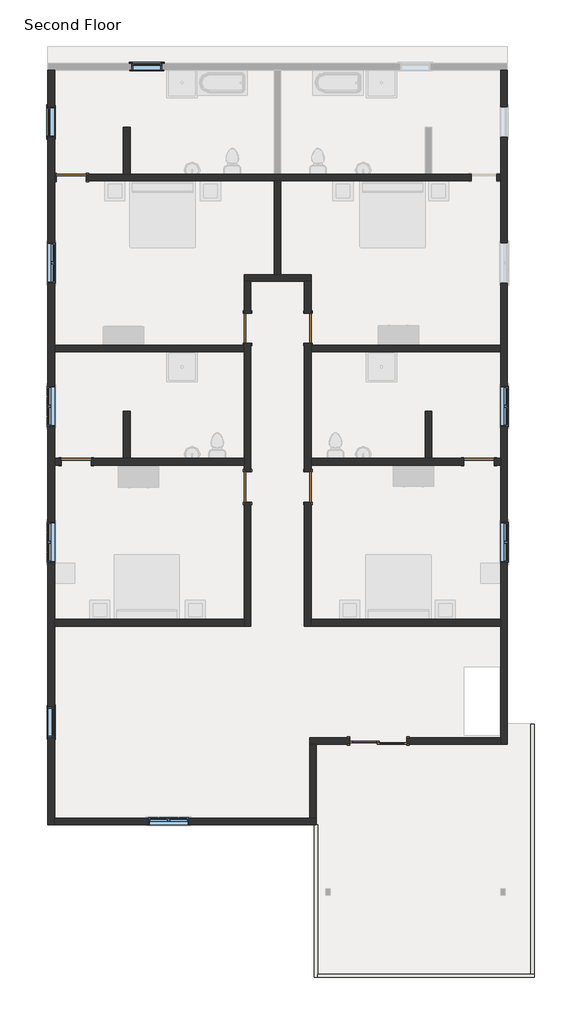
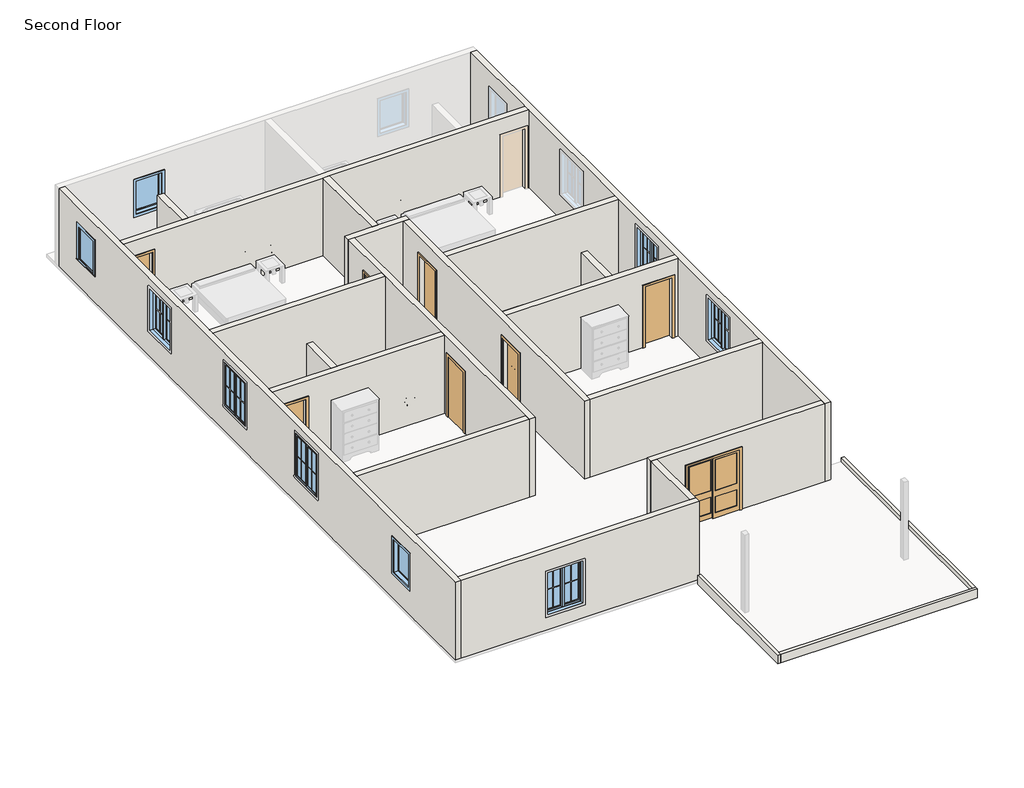
# One storey, part 1 of 2: 22 walls, 9 windows, 8 doors.
"""IFC4 building model written with IfcOpenShell, lengths in millimetres."""

import ifcopenshell
import ifcopenshell.guid

model = None  # the IFC model being written
_history = None  # IfcOwnerHistory: only IFC2X3 demands one
_inside = {}  # id of a spatial element -> (the spatial element, [elements in it])
_under = {}  # id of a project, library or spatial element -> (it, [spatial elements below it])
_declared = {}  # id of a project -> (the project, [libraries it declares])
_typed = {}  # id of a type object -> (the type object, [elements of that type])
_made_of = {}  # id of a material, layer set ... -> (it, [elements and type objects made of it])


def new_model(schema):
    """Start an empty IFC model of exactly this schema.

    Asked for "IFC4X3", IfcOpenShell would pick the latest addendum, in which some entities
    have other attributes; the version numbers below select the first issue.
    IFC2X3 requires an IfcOwnerHistory on every rooted entity: one is made here for all.
    """
    global model, _history
    if schema == "IFC4X3":
        model = ifcopenshell.file(schema_version=(4, 3, 0, 0))
    else:
        model = ifcopenshell.file(schema=schema)
    _inside.clear()
    _under.clear()
    _declared.clear()
    _typed.clear()
    _made_of.clear()
    _history = None
    if model.schema == "IFC2X3":
        org = make("IfcOrganization", Name="unknown")
        user = make(
            "IfcPersonAndOrganization",
            ThePerson=make("IfcPerson", FamilyName="unknown"),
            TheOrganization=org,
        )
        app = make(
            "IfcApplication",
            ApplicationDeveloper=org,
            Version="unknown",
            ApplicationFullName="unknown",
            ApplicationIdentifier="unknown",
        )
        _history = make(
            "IfcOwnerHistory",
            OwningUser=user,
            OwningApplication=app,
            ChangeAction="ADDED",
            CreationDate=0,
        )
    return model


def make(cls, **values):
    """One entity of the class cls with the attributes given. An attribute that is None is left unset."""
    return model.create_entity(
        cls, **{name: value for name, value in values.items() if value is not None}
    )


def rooted(cls, **values):
    """An entity with a GlobalId (a new one), such as an element, a storey or a relation."""
    return make(cls, GlobalId=ifcopenshell.guid.new(), OwnerHistory=_history, **values)


def si_unit(unit_type, name, prefix=None):
    """IfcSIUnit, for example si_unit("LENGTHUNIT", "METRE", prefix="MILLI")."""
    return make("IfcSIUnit", UnitType=unit_type, Prefix=prefix, Name=name)


def assignment(units):
    """IfcUnitAssignment: the units of a project."""
    return None if units is None else make("IfcUnitAssignment", Units=units)


def point(xyz):
    """IfcCartesianPoint."""
    return None if xyz is None else make("IfcCartesianPoint", Coordinates=xyz)


def direction(xyz):
    """IfcDirection."""
    return None if xyz is None else make("IfcDirection", DirectionRatios=xyz)


def frame(location, z_axis=None, x_axis=None):
    """IfcAxis2Placement3D, a coordinate frame: its origin and axes. An axis left out is left unset."""
    return make(
        "IfcAxis2Placement3D",
        Location=point(location),
        Axis=direction(z_axis),
        RefDirection=direction(x_axis),
    )


def origin():
    """The frame at (0, 0, 0) with its axes left unset."""
    return frame((0.0, 0.0, 0.0))


def origin_with_axes():
    """The frame at (0, 0, 0) with the z axis (0, 0, 1) and the x axis (1, 0, 0) written out."""
    return frame((0.0, 0.0, 0.0), z_axis=(0.0, 0.0, 1.0), x_axis=(1.0, 0.0, 0.0))


def place(relative_to, where):
    """IfcLocalPlacement: puts the frame where relative to a parent placement (None: the world)."""
    return make(
        "IfcLocalPlacement", PlacementRelTo=relative_to, RelativePlacement=where
    )


def context(
    kind, dimensions, precision=None, world=None, true_north=None, identifier=None
):
    """IfcGeometricRepresentationContext, for example the 3D "Model" context."""
    return make(
        "IfcGeometricRepresentationContext",
        ContextIdentifier=identifier,
        ContextType=kind,
        CoordinateSpaceDimension=dimensions,
        Precision=precision,
        WorldCoordinateSystem=world,
        TrueNorth=true_north,
    )


def project(units=None, contexts=None):
    """IfcProject with its units and contexts."""
    return rooted(
        "IfcProject",
        Name="project",
        RepresentationContexts=contexts,
        UnitsInContext=assignment(units),
    )


def spatial(cls, under=None, at=None, **own):
    """A site, building, storey or space (cls), placed at a placement, below another one or the project."""
    s = rooted(cls, ObjectPlacement=at, **own)
    if under is not None:
        _under.setdefault(under.id(), (under, []))[1].append(s)
    return s


def polyline(points):
    """IfcPolyline through the points."""
    return make("IfcPolyline", Points=[point(p) for p in points])


def outline(outer, holes=None, kind="AREA"):
    """IfcArbitraryClosedProfileDef: a profile drawn as a closed curve; with holes, ...WithVoids."""
    if holes is None:
        return make("IfcArbitraryClosedProfileDef", ProfileType=kind, OuterCurve=outer)
    return make(
        "IfcArbitraryProfileDefWithVoids",
        ProfileType=kind,
        OuterCurve=outer,
        InnerCurves=holes,
    )


def extrude(swept, where, along, depth):
    """IfcExtrudedAreaSolid: the profile swept, set in the frame where, extruded along a direction by depth."""
    return make(
        "IfcExtrudedAreaSolid",
        SweptArea=swept,
        Position=where,
        ExtrudedDirection=direction(along),
        Depth=depth,
    )


def faces_of(points, faces, orient=None, outer=None):
    """IfcFace entities. A face is a list of loops; a loop is a list of indices into points, from 0.

    orient and outer hold one flag for each loop. By default every Orientation is true, the
    first loop of a face is its IfcFaceOuterBound and the others are IfcFaceBound.
    """
    made = []
    for i, loops in enumerate(faces):
        bounds = []
        for j, loop in enumerate(loops):
            is_outer = j == 0 if outer is None else outer[i][j]
            bounds.append(
                make(
                    "IfcFaceOuterBound" if is_outer else "IfcFaceBound",
                    Bound=make("IfcPolyLoop", Polygon=[points[k] for k in loop]),
                    Orientation=True if orient is None else orient[i][j],
                )
            )
        made.append(make("IfcFace", Bounds=bounds))
    return made


def faceted_brep(points, faces, orient=None, outer=None, voids=None):
    """IfcFacetedBrep: a solid bounded by flat faces; with voids (closed shells), ...WithVoids."""
    shared = [point(p) for p in points]
    hull = make("IfcClosedShell", CfsFaces=faces_of(shared, faces, orient, outer))
    if voids is None:
        return make("IfcFacetedBrep", Outer=hull)
    return make(
        "IfcFacetedBrepWithVoids",
        Outer=hull,
        Voids=[
            make(cls, CfsFaces=faces_of(shared, fs, o, b)) for cls, fs, o, b in voids
        ],
    )


def shape(context_of_items, identifier, shape_type, items):
    """IfcShapeRepresentation: the items that make up one representation, for example the "Body"."""
    return make(
        "IfcShapeRepresentation",
        ContextOfItems=context_of_items,
        RepresentationIdentifier=identifier,
        RepresentationType=shape_type,
        Items=items,
    )


def source(mapping_origin, context_of_items, identifier, shape_type, items):
    """IfcRepresentationMap: a shape defined once, which mapped items show again and again."""
    return make(
        "IfcRepresentationMap",
        MappingOrigin=mapping_origin,
        MappedRepresentation=shape(context_of_items, identifier, shape_type, items),
    )


def transform(
    local_origin,
    x_axis=None,
    y_axis=None,
    z_axis=None,
    scale=None,
    scale2=None,
    scale3=None,
    uniform=True,
):
    """IfcCartesianTransformationOperator3D, or its non-uniform kind. x_axis, y_axis, z_axis: its Axis1, 2, 3."""
    if uniform:
        return make(
            "IfcCartesianTransformationOperator3D",
            Axis1=direction(x_axis),
            Axis2=direction(y_axis),
            LocalOrigin=point(local_origin),
            Scale=scale,
            Axis3=direction(z_axis),
        )
    return make(
        "IfcCartesianTransformationOperator3DnonUniform",
        Axis1=direction(x_axis),
        Axis2=direction(y_axis),
        LocalOrigin=point(local_origin),
        Scale=scale,
        Axis3=direction(z_axis),
        Scale2=scale2,
        Scale3=scale3,
    )


def mapped(mapping_source, mapping_target):
    """IfcMappedItem: shows the shape of a source again, moved by a transform."""
    return make(
        "IfcMappedItem", MappingSource=mapping_source, MappingTarget=mapping_target
    )


def made_of(thing, what):
    """Note that an element or type object is made of a material, layer set ...; save() writes the relation."""
    if what is not None:
        _made_of.setdefault(what.id(), (what, []))[1].append(thing)
    return thing


def element(
    cls,
    number,
    at=None,
    inside=None,
    cuts=None,
    type_object=None,
    material=None,
    context=None,
    identifier="Body",
    shape_type=None,
    held_by="IfcProductDefinitionShape",
    body=None,
    shapes=None,
    **own,
):
    """One element of the class cls, such as IfcWall. Its Tag is "e" and its number.

    at: its placement. inside: the storey or other place that contains it. cuts: it is an
    opening in that element (IfcRelVoidsElement). A single representation is given by context,
    identifier, shape_type and body (its items); several are given by shapes. held_by: the class
    of the entity that holds the representations. save() writes the other relations.
    """
    e = rooted(cls, Tag="e%d" % number, ObjectPlacement=at, **own)
    if body is not None:
        shapes = [shape(context, identifier, shape_type, body)]
    if shapes is not None:
        e.Representation = make(held_by, Representations=shapes)
    if inside is not None:
        _inside.setdefault(inside.id(), (inside, []))[1].append(e)
    if cuts is not None:
        rooted(
            "IfcRelVoidsElement", RelatingBuildingElement=cuts, RelatedOpeningElement=e
        )
    if type_object is not None:
        _typed.setdefault(type_object.id(), (type_object, []))[1].append(e)
    return made_of(e, material)


def aggregate(whole, parts):
    """IfcRelAggregates: a whole, such as a stair, and the parts it consists of."""
    return rooted("IfcRelAggregates", RelatingObject=whole, RelatedObjects=parts)


def save(model, path):
    """Write the relations noted so far, then the file.

    IfcRelAggregates (storeys below a building ...), IfcRelContainedInSpatialStructure (elements
    in a storey), IfcRelDefinesByType, IfcRelAssociatesMaterial and IfcRelDeclares: one each for
    every whole, place, type object, material and project.
    """
    for whole, parts in _under.values():
        aggregate(whole, parts)
    for where, things in _inside.values():
        rooted(
            "IfcRelContainedInSpatialStructure",
            RelatedElements=things,
            RelatingStructure=where,
        )
    for kind, things in _typed.values():
        rooted("IfcRelDefinesByType", RelatedObjects=things, RelatingType=kind)
    for what, things in _made_of.values():
        rooted("IfcRelAssociatesMaterial", RelatedObjects=things, RelatingMaterial=what)
    for by, libraries in _declared.values():
        rooted("IfcRelDeclares", RelatingContext=by, RelatedDefinitions=libraries)
    model.write(path)


def door_54dd4da4(model_context):
    return source(origin(), model_context, "Body", "SweptSolid", [
        extrude(outline(polyline([(2209.8, -533.4), (0.0, -533.4), (0.0, -457.2), (2133.6, -457.2), (2133.6, 457.2), (0.0, 457.2), (0.0, 533.4), (2209.8, 533.4), (2209.8, -533.4)])), frame((0.0, 101.6, 0.0), z_axis=(0.0, 1.0, 0.0), x_axis=(0.0, 0.0, 1.0)), (0.0, 0.0, 1.0), 25.4),
        extrude(outline(polyline([(2209.8, 533.4), (2209.8, -533.4), (0.0, -533.4), (0.0, -457.2), (2133.6, -457.2), (2133.6, 457.2), (0.0, 457.2), (0.0, 533.4), (2209.8, 533.4)])), frame((0.0, -127.0, 0.0), z_axis=(0.0, 1.0, 0.0), x_axis=(0.0, 0.0, 1.0)), (0.0, 0.0, 1.0), 25.4),
        extrude(outline(polyline([(457.2, 50.8), (-457.2, 50.8), (-457.2, 101.6), (457.2, 101.6), (457.2, 50.8)])), origin_with_axes(), (0.0, 0.0, 1.0), 2133.6),
    ])


def door_719f80de(model_context):
    return source(origin(), model_context, "Body", "SweptSolid", [
        extrude(outline(polyline([(2209.8, -533.4), (0.0, -533.4), (0.0, -457.2), (2133.6, -457.2), (2133.6, 457.2), (0.0, 457.2), (0.0, 533.4), (2209.8, 533.4), (2209.8, -533.4)])), frame((0.0, -127.0, 0.0), z_axis=(0.0, 1.0, 0.0), x_axis=(0.0, 0.0, 1.0)), (0.0, 0.0, 1.0), 25.4),
        extrude(outline(polyline([(2209.8, 533.4), (2209.8, -533.4), (0.0, -533.4), (0.0, -457.2), (2133.6, -457.2), (2133.6, 457.2), (0.0, 457.2), (0.0, 533.4), (2209.8, 533.4)])), frame((0.0, 101.6, 0.0), z_axis=(0.0, 1.0, 0.0), x_axis=(0.0, 0.0, 1.0)), (0.0, 0.0, 1.0), 25.4),
        extrude(outline(polyline([(457.2, -50.8), (457.2, -101.6), (-457.2, -101.6), (-457.2, -50.8), (457.2, -50.8)])), origin_with_axes(), (0.0, 0.0, 1.0), 2133.6),
    ])


def door_2f313a91(model_context):
    return source(origin(), model_context, "Body", "SweptSolid", [
        extrude(outline(polyline([(-63.5, 190.5), (-774.7, 190.5), (-774.7, 215.9), (-63.5, 215.9), (-63.5, 190.5)])), frame((0.0, 0.0, 965.2), z_axis=(0.0, 0.0, 1.0), x_axis=(1.0, 0.0, 0.0)), (0.0, 0.0, 1.0), 1079.5),
        extrude(outline(polyline([(-63.5, 190.5), (-774.7, 190.5), (-774.7, 215.9), (-63.5, 215.9), (-63.5, 190.5)])), frame((0.0, 0.0, 184.15), z_axis=(0.0, 0.0, 1.0), x_axis=(1.0, 0.0, 0.0)), (0.0, 0.0, 1.0), 565.15),
        extrude(outline(polyline([(63.5, 165.1), (774.7, 165.1), (774.7, 139.7), (63.5, 139.7), (63.5, 165.1)])), frame((0.0, 0.0, 965.2), z_axis=(0.0, 0.0, 1.0), x_axis=(1.0, 0.0, 0.0)), (0.0, 0.0, 1.0), 1079.5),
        extrude(outline(polyline([(63.5, 165.1), (774.7, 165.1), (774.7, 139.7), (63.5, 139.7), (63.5, 165.1)])), frame((0.0, 0.0, 184.15), z_axis=(0.0, 0.0, 1.0), x_axis=(1.0, 0.0, 0.0)), (0.0, 0.0, 1.0), 565.15),
        extrude(outline(polyline([(2133.6, 25.4), (2133.6, -863.6), (0.0, -863.6), (0.0, 25.4), (2133.6, 25.4)]), holes=[polyline([(184.15, -774.7), (749.3, -774.7), (749.3, -63.5), (184.15, -63.5), (184.15, -774.7)]), polyline([(965.2, -774.7), (2044.7, -774.7), (2044.7, -63.5), (965.2, -63.5), (965.2, -774.7)])]), frame((0.0, 177.8, 0.0), z_axis=(0.0, 1.0, 0.0), x_axis=(0.0, 0.0, 1.0)), (0.0, 0.0, 1.0), 50.8),
        extrude(outline(polyline([(0.0, -939.8), (0.0, -863.6), (2133.6, -863.6), (2133.6, 863.6), (0.0, 863.6), (0.0, 939.8), (2209.8, 939.8), (2209.8, -939.8), (0.0, -939.8)])), frame((0.0, 0.0, 0.0), z_axis=(0.0, 1.0, 0.0), x_axis=(0.0, 0.0, 1.0)), (0.0, 0.0, 1.0), 25.4),
        extrude(outline(polyline([(0.0, 939.8), (2209.8, 939.8), (2209.8, -939.8), (0.0, -939.8), (0.0, -863.6), (2133.6, -863.6), (2133.6, 863.6), (0.0, 863.6), (0.0, 939.8)])), frame((0.0, 228.6, 0.0), z_axis=(0.0, 1.0, 0.0), x_axis=(0.0, 0.0, 1.0)), (0.0, 0.0, 1.0), 25.4),
        extrude(outline(polyline([(2133.6, -25.4), (0.0, -25.4), (0.0, 863.6), (2133.6, 863.6), (2133.6, -25.4)]), holes=[polyline([(965.2, 774.7), (965.2, 63.5), (2044.7, 63.5), (2044.7, 774.7), (965.2, 774.7)]), polyline([(184.15, 774.7), (184.15, 63.5), (749.3, 63.5), (749.3, 774.7), (184.15, 774.7)])]), frame((0.0, 127.0, 0.0), z_axis=(0.0, 1.0, 0.0), x_axis=(0.0, 0.0, 1.0)), (0.0, 0.0, 1.0), 50.8),
    ])


def window_bec2521a(model_context):
    return source(origin(), model_context, "Body", "SweptSolid", [
        extrude(outline(polyline([(-565.15, 127.0), (488.95, 127.0), (488.95, 101.6), (-565.15, 101.6), (-565.15, 127.0)])), frame((0.0, 0.0, 914.4), z_axis=(0.0, 0.0, 1.0), x_axis=(1.0, 0.0, 0.0)), (0.0, 0.0, 1.0), 19.05),
        extrude(outline(polyline([(2114.55, -476.25), (2114.55, 400.05), (933.45, 400.05), (933.45, 488.95), (2203.45, 488.95), (2203.45, -565.15), (933.45, -565.15), (933.45, -476.25), (2114.55, -476.25)])), frame((0.0, 101.6, 0.0), z_axis=(0.0, 1.0, 0.0), x_axis=(0.0, 0.0, 1.0)), (0.0, 0.0, 1.0), 12.7),
        extrude(outline(polyline([(2190.75, 476.25), (2190.75, -552.45), (857.25, -552.45), (857.25, 476.25), (2190.75, 476.25)]), holes=[polyline([(2101.85, 387.35), (946.15, 387.35), (946.15, -463.55), (2101.85, -463.55), (2101.85, 387.35)])]), frame((0.0, -120.65, 0.0), z_axis=(0.0, 1.0, 0.0), x_axis=(0.0, 0.0, 1.0)), (0.0, 0.0, 1.0), 19.05),
        extrude(outline(polyline([(355.6, 53.975), (-431.8, 53.975), (-431.8, 66.675), (355.6, 66.675), (355.6, 53.975)])), frame((0.0, 0.0, 977.9), z_axis=(0.0, 0.0, 1.0), x_axis=(1.0, 0.0, 0.0)), (0.0, 0.0, 1.0), 1092.2),
        extrude(outline(polyline([(2114.55, -476.25), (933.45, -476.25), (933.45, 400.05), (2114.55, 400.05), (2114.55, -476.25)]), holes=[polyline([(2070.1, -431.8), (2070.1, 355.6), (977.9, 355.6), (977.9, -431.8), (2070.1, -431.8)])]), frame((0.0, 38.1, 0.0), z_axis=(0.0, 1.0, 0.0), x_axis=(0.0, 0.0, 1.0)), (0.0, 0.0, 1.0), 44.45),
        extrude(outline(polyline([(2133.6, -495.3), (914.4, -495.3), (914.4, 419.1), (2133.6, 419.1), (2133.6, -495.3)]), holes=[polyline([(2101.85, -463.55), (2101.85, 387.35), (946.15, 387.35), (946.15, -463.55), (2101.85, -463.55)])]), frame((0.0, -101.6, 0.0), z_axis=(0.0, 1.0, 0.0), x_axis=(0.0, 0.0, 1.0)), (0.0, 0.0, 1.0), 139.7),
        extrude(outline(polyline([(2133.6, 419.1), (2133.6, -495.3), (914.4, -495.3), (914.4, 419.1), (2133.6, 419.1)]), holes=[polyline([(2114.55, 400.05), (933.45, 400.05), (933.45, -476.25), (2114.55, -476.25), (2114.55, 400.05)])]), frame((0.0, 38.1, 0.0), z_axis=(0.0, 1.0, 0.0), x_axis=(0.0, 0.0, 1.0)), (0.0, 0.0, 1.0), 63.5),
    ])


def window_78633f8a(model_context):
    return source(origin(), model_context, "Body", "SolidModel", [
        faceted_brep([(9.525, 120.65, 2425.7), (-9.525, 120.65, 2425.7), (-9.525, 69.85, 2425.7), (9.525, 69.85, 2425.7), (9.525, 120.65, 927.1), (9.525, 69.85, 927.1), (-9.525, 69.85, 927.1), (-9.525, 120.65, 927.1), (-9.525, 69.85, 946.15), (-9.525, 69.85, 2406.65), (-30.1625, 69.85, 946.15), (-30.1625, 69.85, 2406.65), (-30.1625, 6.35, 946.15), (-30.1625, 6.35, 2406.65), (30.1625, 6.35, 946.15), (30.1625, 6.35, 2406.65), (30.1625, 69.85, 946.15), (30.1625, 69.85, 2406.65), (9.525, 69.85, 946.15), (9.525, 69.85, 2406.65)], [[[0, 1, 2, 3]], [[4, 5, 6, 7]], [[1, 0, 4, 7]], [[2, 1, 7, 6, 8, 9]], [[9, 8, 10, 11]], [[11, 10, 12, 13]], [[13, 12, 14, 15]], [[15, 14, 16, 17]], [[17, 16, 18, 19]], [[0, 3, 19, 18, 5, 4]], [[18, 8, 6, 5]], [[9, 19, 3, 2]], [[8, 18, 16, 14, 12, 10]], [[19, 9, 11, 13, 15, 17]]]),
        extrude(outline(polyline([(-66.675, 101.6), (-66.675, 95.25), (-539.75, 95.25), (-539.75, 101.6), (-66.675, 101.6)])), frame((0.0, 0.0, 984.25), z_axis=(0.0, 0.0, 1.0), x_axis=(1.0, 0.0, 0.0)), (0.0, 0.0, 1.0), 1384.3),
        extrude(outline(polyline([(-539.75, 82.55), (-539.75, 88.9), (-66.675, 88.9), (-66.675, 82.55), (-539.75, 82.55)])), frame((0.0, 0.0, 984.25), z_axis=(0.0, 0.0, 1.0), x_axis=(1.0, 0.0, 0.0)), (0.0, 0.0, 1.0), 1384.3),
        extrude(outline(polyline([(539.75, 101.6), (539.75, 95.25), (66.675, 95.25), (66.675, 101.6), (539.75, 101.6)])), frame((0.0, 0.0, 984.25), z_axis=(0.0, 0.0, 1.0), x_axis=(1.0, 0.0, 0.0)), (0.0, 0.0, 1.0), 1384.3),
        extrude(outline(polyline([(66.675, 82.55), (66.675, 88.9), (539.75, 88.9), (539.75, 82.55), (66.675, 82.55)])), frame((0.0, 0.0, 984.25), z_axis=(0.0, 0.0, 1.0), x_axis=(1.0, 0.0, 0.0)), (0.0, 0.0, 1.0), 1384.3),
        extrude(outline(polyline([(2425.7, -596.9), (927.1, -596.9), (927.1, -9.525), (2425.7, -9.525), (2425.7, -596.9)]), holes=[polyline([(2368.55, -66.675), (984.25, -66.675), (984.25, -539.75), (2368.55, -539.75), (2368.55, -66.675)])]), frame((0.0, 69.85, 0.0), z_axis=(0.0, 1.0, 0.0), x_axis=(0.0, 0.0, 1.0)), (0.0, 0.0, 1.0), 44.45),
        extrude(outline(polyline([(927.1, 596.9), (2425.7, 596.9), (2425.7, 9.525), (927.1, 9.525), (927.1, 596.9)]), holes=[polyline([(984.25, 66.675), (2368.55, 66.675), (2368.55, 539.75), (984.25, 539.75), (984.25, 66.675)])]), frame((0.0, 69.85, 0.0), z_axis=(0.0, 1.0, 0.0), x_axis=(0.0, 0.0, 1.0)), (0.0, 0.0, 1.0), 44.45),
        extrude(outline(polyline([(2438.4, -609.6), (914.4, -609.6), (914.4, 609.6), (2438.4, 609.6), (2438.4, -609.6)]), holes=[polyline([(2419.35, 590.55), (933.45, 590.55), (933.45, -590.55), (2419.35, -590.55), (2419.35, 590.55)])]), frame((0.0, -101.6, 0.0), z_axis=(0.0, 1.0, 0.0), x_axis=(0.0, 0.0, 1.0)), (0.0, 0.0, 1.0), 107.95),
        faceted_brep([(577.85, 69.85, 2406.65), (577.85, 6.35, 2406.65), (-577.85, 6.35, 2406.65), (-577.85, 69.85, 2406.65), (596.9, 120.65, 2425.7), (596.9, 69.85, 2425.7), (-596.9, 69.85, 2425.7), (-596.9, 120.65, 2425.7), (609.6, 6.35, 2438.4), (609.6, 120.65, 2438.4), (-609.6, 120.65, 2438.4), (-609.6, 6.35, 2438.4), (-577.85, 6.35, 946.15), (-577.85, 69.85, 946.15), (-596.9, 69.85, 927.1), (-596.9, 120.65, 927.1), (-609.6, 120.65, 914.4), (-609.6, 6.35, 914.4), (577.85, 6.35, 946.15), (577.85, 69.85, 946.15), (596.9, 69.85, 927.1), (596.9, 120.65, 927.1), (609.6, 120.65, 914.4), (609.6, 6.35, 914.4)], [[[0, 1, 2, 3]], [[4, 5, 6, 7]], [[8, 9, 10, 11]], [[3, 2, 12, 13]], [[7, 6, 14, 15]], [[11, 10, 16, 17]], [[13, 12, 18, 19]], [[15, 14, 20, 21]], [[17, 16, 22, 23]], [[11, 17, 23, 8], [1, 18, 12, 2]], [[19, 18, 1, 0]], [[5, 20, 14, 6], [3, 13, 19, 0]], [[21, 20, 5, 4]], [[23, 22, 9, 8]], [[9, 22, 16, 10], [7, 15, 21, 4]]]),
    ])


model = new_model("IFC4")

# Units and contexts
model_context = context("Model", 3, world=origin())
ifc_project = project(units=[si_unit("LENGTHUNIT", "METRE", prefix="MILLI")], contexts=[model_context])

# Site, building, storey
site = spatial("IfcSite", under=ifc_project)
building = spatial("IfcBuilding", under=site)
storey = spatial("IfcBuildingStorey", under=building, Name="Second Floor", Elevation=2743.2)

# Doors
placement = place(None, origin())
door_shape = door_54dd4da4(model_context)
element("IfcDoor", 1, ObjectType="Single-Flush : 36\" x 84\"", at=placement, inside=storey, context=model_context, shape_type="MappedRepresentation", body=[
    mapped(door_shape, transform((-5575.1210655, 3585.6263295, 2743.2), x_axis=(1.0, 0.0, 0.0), y_axis=(0.0, 1.0, 0.0), z_axis=(0.0, 0.0, 1.0))),
])
element("IfcDoor", 2, ObjectType="Single-Flush : 36\" x 84\"", at=placement, inside=storey, context=model_context, shape_type="MappedRepresentation", body=[
    mapped(door_shape, transform((1587.6789345, -986.3736705, 2743.2), x_axis=(0.0, -1.0, 0.0), y_axis=(1.0, 0.0, 0.0), z_axis=(0.0, 0.0, 1.0))),
])
element("IfcDoor", 3, ObjectType="Single-Flush : 36\" x 84\"", at=placement, inside=storey, context=model_context, shape_type="MappedRepresentation", body=[
    mapped(door_shape, transform((-5422.7210655, -5024.9736705, 2743.2), x_axis=(1.0, 0.0, 0.0), y_axis=(0.0, 1.0, 0.0), z_axis=(0.0, 0.0, 1.0))),
])
element("IfcDoor", 4, ObjectType="Single-Flush : 36\" x 84\"", at=placement, inside=storey, context=model_context, shape_type="MappedRepresentation", body=[
    mapped(door_shape, transform((-241.1210655, -5786.9736705, 2743.2), x_axis=(0.0, 1.0, 0.0), y_axis=(-1.0, 0.0, 0.0), z_axis=(0.0, 0.0, 1.0))),
])
door_2_shape = door_719f80de(model_context)
element("IfcDoor", 5, ObjectType="Single-Flush : 36\" x 84\"", at=placement, inside=storey, context=model_context, shape_type="MappedRepresentation", body=[
    mapped(door_2_shape, transform((6769.2789345, -5024.9736705, 2743.2), x_axis=(-1.0, 0.0, 0.0), y_axis=(0.0, -1.0, 0.0), z_axis=(0.0, 0.0, 1.0))),
])
element("IfcDoor", 6, ObjectType="Single-Flush : 36\" x 84\"", at=placement, inside=storey, context=model_context, shape_type="MappedRepresentation", body=[
    mapped(door_2_shape, transform((-241.1210655, -986.3736705, 2743.2), x_axis=(0.0, -1.0, 0.0), y_axis=(1.0, 0.0, 0.0), z_axis=(0.0, 0.0, 1.0))),
])
element("IfcDoor", 7, ObjectType="Single-Flush : 36\" x 84\"", at=placement, inside=storey, context=model_context, shape_type="MappedRepresentation", body=[
    mapped(door_2_shape, transform((1587.6789345, -5786.9736705, 2743.2), x_axis=(0.0, 1.0, 0.0), y_axis=(-1.0, 0.0, 0.0), z_axis=(0.0, 0.0, 1.0))),
])
door_3_shape = door_2f313a91(model_context)
element("IfcDoor", 8, ObjectType="Sliding-Closet : 68\" x 84\"", at=placement, inside=storey, context=model_context, shape_type="MappedRepresentation", body=[
    mapped(door_3_shape, transform((3721.2789345, -13356.1736705, 2743.2), x_axis=(-1.0, 0.0, 0.0), y_axis=(0.0, -1.0, 0.0), z_axis=(0.0, 0.0, 1.0))),
])

# Walls
element("IfcWall", 9, ObjectType="Generic - 4\"", at=placement, inside=storey, context=model_context, shape_type="Brep", body=[
    faceted_brep([(1786.1164345, -16023.1736705, 2590.8), (1786.1164345, -20641.2111705, 2590.8), (1786.1164345, -20641.2111705, 2895.6), (1786.1164345, -16023.1736705, 2895.6), (1887.7164345, -16023.1736705, 2590.8), (1887.7164345, -16023.1736705, 2895.6), (1887.7164345, -20539.6111705, 2895.6), (1887.7164345, -20641.2111705, 2895.6), (1887.7164345, -20641.2111705, 2590.8), (1887.7164345, -20539.6111705, 2590.8)], [[[0, 1, 2, 3]], [[4, 5, 6, 7, 8, 9]], [[1, 0, 4, 9, 8]], [[3, 2, 7, 6, 5]], [[0, 3, 5, 4]], [[2, 1, 8, 7]]]),
])
element("IfcWall", 10, ObjectType="Generic - 4\"", at=placement, inside=storey, context=model_context, shape_type="Brep", body=[
    faceted_brep([(1887.7164345, -20641.2111705, 2590.8), (8440.9164345, -20641.2111705, 2590.8), (8440.9164345, -20641.2111705, 2895.6), (1887.7164345, -20641.2111705, 2895.6), (1887.7164345, -20539.6111705, 2590.8), (1887.7164345, -20539.6111705, 2895.6), (8339.3164345, -20539.6111705, 2895.6), (8440.9164345, -20539.6111705, 2895.6), (8440.9164345, -20539.6111705, 2590.8), (8339.3164345, -20539.6111705, 2590.8)], [[[0, 1, 2, 3]], [[4, 5, 6, 7, 8, 9]], [[1, 0, 4, 9, 8]], [[3, 2, 7, 6, 5]], [[0, 3, 5, 4]], [[2, 1, 8, 7]]]),
])
element("IfcWall", 11, ObjectType="Generic - 4\"", at=placement, inside=storey, context=model_context, shape_type="SweptSolid", body=[
    extrude(outline(polyline([(8440.9164345, -12970.4111705), (8440.9164345, -20539.6111705), (8339.3164345, -20539.6111705), (8339.3164345, -12970.4111705), (8440.9164345, -12970.4111705)])), frame((0.0, 0.0, 2590.8), z_axis=(0.0, 0.0, 1.0), x_axis=(1.0, 0.0, 0.0)), (0.0, 0.0, 1.0), 304.8),
])
element("IfcWall", 12, ObjectType="Generic - 8\" - Filled", at=placement, inside=storey, context=model_context, shape_type="Brep", body=[
    faceted_brep([(7429.6789345, 6836.8263295, 2743.2), (7429.6789345, 3687.2263295, 2743.2), (7429.6789345, 3484.0263295, 2743.2), (7429.6789345, -1494.3736705, 2743.2), (7429.6789345, -1697.5736705, 2743.2), (7429.6789345, -4923.3736705, 2743.2), (7429.6789345, -5126.5736705, 2743.2), (7429.6789345, -9800.1736705, 2743.2), (7429.6789345, -10003.3736705, 2743.2), (7429.6789345, -13381.5736705, 2743.2), (7429.6789345, -13584.7736705, 2743.2), (7429.6789345, -13584.7736705, 5486.4), (7429.6789345, -13381.5736705, 5486.4), (7429.6789345, -10003.3736705, 5486.4), (7429.6789345, -9800.1736705, 5486.4), (7429.6789345, -5126.5736705, 5486.4), (7429.6789345, -4923.3736705, 5486.4), (7429.6789345, -1697.5736705, 5486.4), (7429.6789345, -1494.3736705, 5486.4), (7429.6789345, 3484.0263295, 5486.4), (7429.6789345, 3687.2263295, 5486.4), (7429.6789345, 6836.8263295, 5486.4), (7429.6789345, 4804.8263295, 4876.8), (7429.6789345, 4804.8263295, 3657.6), (7429.6789345, 5719.2263295, 3657.6), (7429.6789345, 5719.2263295, 4876.8), (7429.6789345, -3958.1736705, 5181.6), (7429.6789345, -3958.1736705, 3657.6), (7429.6789345, -2738.9736705, 3657.6), (7429.6789345, -2738.9736705, 5181.6), (7429.6789345, -8072.9736705, 5181.6), (7429.6789345, -8072.9736705, 3657.6), (7429.6789345, -6853.7736705, 3657.6), (7429.6789345, -6853.7736705, 5181.6), (7429.6789345, 385.2263295, 5181.6), (7429.6789345, 385.2263295, 3657.6), (7429.6789345, 1604.4263295, 3657.6), (7429.6789345, 1604.4263295, 5181.6), (7632.8789345, 6836.8263295, 2743.2), (7632.8789345, 6836.8263295, 5486.4), (7632.8789345, -13584.7736705, 5486.4), (7632.8789345, -13584.7736705, 2743.2), (7632.8789345, 4804.8263295, 4876.8), (7632.8789345, 5719.2263295, 4876.8), (7632.8789345, 5719.2263295, 3657.6), (7632.8789345, 4804.8263295, 3657.6), (7632.8789345, -3958.1736705, 5181.6), (7632.8789345, -2738.9736705, 5181.6), (7632.8789345, -2738.9736705, 3657.6), (7632.8789345, -3958.1736705, 3657.6), (7632.8789345, -8072.9736705, 5181.6), (7632.8789345, -6853.7736705, 5181.6), (7632.8789345, -6853.7736705, 3657.6), (7632.8789345, -8072.9736705, 3657.6), (7632.8789345, 385.2263295, 5181.6), (7632.8789345, 1604.4263295, 5181.6), (7632.8789345, 1604.4263295, 3657.6), (7632.8789345, 385.2263295, 3657.6)], [[[0, 1, 2, 3, 4, 5, 6, 7, 8, 9, 10, 11, 12, 13, 14, 15, 16, 17, 18, 19, 20, 21], [22, 23, 24, 25], [26, 27, 28, 29], [30, 31, 32, 33], [34, 35, 36, 37]], [[38, 39, 40, 41], [42, 43, 44, 45], [46, 47, 48, 49], [50, 51, 52, 53], [54, 55, 56, 57]], [[10, 9, 8, 7, 6, 5, 4, 3, 2, 1, 0, 38, 41]], [[21, 20, 19, 18, 17, 16, 15, 14, 13, 12, 11, 40, 39]], [[0, 21, 39, 38]], [[23, 22, 42, 45]], [[24, 23, 45, 44]], [[25, 24, 44, 43]], [[22, 25, 43, 42]], [[27, 26, 46, 49]], [[28, 27, 49, 48]], [[29, 28, 48, 47]], [[26, 29, 47, 46]], [[11, 10, 41, 40]], [[31, 30, 50, 53]], [[32, 31, 53, 52]], [[33, 32, 52, 51]], [[30, 33, 51, 50]], [[35, 34, 54, 57]], [[36, 35, 57, 56]], [[37, 36, 56, 55]], [[34, 37, 55, 54]]]),
])
element("IfcWall", 13, ObjectType="Generic - 8\" - Filled", at=placement, inside=storey, context=model_context, shape_type="Brep", body=[
    faceted_brep([(-6083.1210655, -16023.1736705, 2743.2), (-6083.1210655, -15819.9736705, 2743.2), (-6083.1210655, -10003.3736705, 2743.2), (-6083.1210655, -9800.1736705, 2743.2), (-6083.1210655, -5126.5736705, 2743.2), (-6083.1210655, -4923.3736705, 2743.2), (-6083.1210655, -1697.5736705, 2743.2), (-6083.1210655, -1494.3736705, 2743.2), (-6083.1210655, 3484.0263295, 2743.2), (-6083.1210655, 3687.2263295, 2743.2), (-6083.1210655, 6836.8263295, 2743.2), (-6083.1210655, 6836.8263295, 5486.4), (-6083.1210655, 3687.2263295, 5486.4), (-6083.1210655, 3484.0263295, 5486.4), (-6083.1210655, -1494.3736705, 5486.4), (-6083.1210655, -1697.5736705, 5486.4), (-6083.1210655, -4923.3736705, 5486.4), (-6083.1210655, -5126.5736705, 5486.4), (-6083.1210655, -9800.1736705, 5486.4), (-6083.1210655, -10003.3736705, 5486.4), (-6083.1210655, -15819.9736705, 5486.4), (-6083.1210655, -16023.1736705, 5486.4), (-6083.1210655, 5719.2263295, 4876.8), (-6083.1210655, 5719.2263295, 3657.6), (-6083.1210655, 4804.8263295, 3657.6), (-6083.1210655, 4804.8263295, 4876.8), (-6083.1210655, -2738.9736705, 5181.6), (-6083.1210655, -2738.9736705, 3657.6), (-6083.1210655, -3958.1736705, 3657.6), (-6083.1210655, -3958.1736705, 5181.6), (-6083.1210655, -6853.7736705, 5181.6), (-6083.1210655, -6853.7736705, 3657.6), (-6083.1210655, -8072.9736705, 3657.6), (-6083.1210655, -8072.9736705, 5181.6), (-6083.1210655, -13368.8736705, 4876.8), (-6083.1210655, -12454.4736705, 4876.8), (-6083.1210655, -12454.4736705, 3657.6), (-6083.1210655, -13368.8736705, 3657.6), (-6083.1210655, 385.2263295, 5181.6), (-6083.1210655, 1604.4263295, 5181.6), (-6083.1210655, 1604.4263295, 3657.6), (-6083.1210655, 385.2263295, 3657.6), (-6286.3210655, -16023.1736705, 2743.2), (-6286.3210655, -16023.1736705, 5486.4), (-6286.3210655, 6836.8263295, 5486.4), (-6286.3210655, 6836.8263295, 2743.2), (-6286.3210655, 5719.2263295, 4876.8), (-6286.3210655, 4804.8263295, 4876.8), (-6286.3210655, 4804.8263295, 3657.6), (-6286.3210655, 5719.2263295, 3657.6), (-6286.3210655, -2738.9736705, 5181.6), (-6286.3210655, -3958.1736705, 5181.6), (-6286.3210655, -3958.1736705, 3657.6), (-6286.3210655, -2738.9736705, 3657.6), (-6286.3210655, -6853.7736705, 5181.6), (-6286.3210655, -8072.9736705, 5181.6), (-6286.3210655, -8072.9736705, 3657.6), (-6286.3210655, -6853.7736705, 3657.6), (-6286.3210655, -13368.8736705, 4876.8), (-6286.3210655, -13368.8736705, 3657.6), (-6286.3210655, -12454.4736705, 3657.6), (-6286.3210655, -12454.4736705, 4876.8), (-6286.3210655, 385.2263295, 5181.6), (-6286.3210655, 385.2263295, 3657.6), (-6286.3210655, 1604.4263295, 3657.6), (-6286.3210655, 1604.4263295, 5181.6)], [[[0, 1, 2, 3, 4, 5, 6, 7, 8, 9, 10, 11, 12, 13, 14, 15, 16, 17, 18, 19, 20, 21], [22, 23, 24, 25], [26, 27, 28, 29], [30, 31, 32, 33], [34, 35, 36, 37], [38, 39, 40, 41]], [[42, 43, 44, 45], [46, 47, 48, 49], [50, 51, 52, 53], [54, 55, 56, 57], [58, 59, 60, 61], [62, 63, 64, 65]], [[10, 9, 8, 7, 6, 5, 4, 3, 2, 1, 0, 42, 45]], [[21, 20, 19, 18, 17, 16, 15, 14, 13, 12, 11, 44, 43]], [[11, 10, 45, 44]], [[23, 22, 46, 49]], [[24, 23, 49, 48]], [[25, 24, 48, 47]], [[22, 25, 47, 46]], [[0, 21, 43, 42]], [[27, 26, 50, 53]], [[28, 27, 53, 52]], [[29, 28, 52, 51]], [[26, 29, 51, 50]], [[31, 30, 54, 57]], [[32, 31, 57, 56]], [[33, 32, 56, 55]], [[30, 33, 55, 54]], [[59, 58, 34, 37]], [[60, 59, 37, 36]], [[61, 60, 36, 35]], [[58, 61, 35, 34]], [[63, 62, 38, 41]], [[64, 63, 41, 40]], [[65, 64, 40, 39]], [[62, 65, 39, 38]]]),
])
element("IfcWall", 14, ObjectType="Generic - 8\" - Filled", at=placement, inside=storey, context=model_context, shape_type="Brep", body=[
    faceted_brep([(-5117.9210655, 3484.0263295, 2743.2), (571.6789345, 3484.0263295, 2743.2), (774.8789345, 3484.0263295, 2743.2), (6540.6789345, 3484.0263295, 2743.2), (6540.6789345, 3484.0263295, 4876.8), (7302.6789345, 3484.0263295, 4876.8), (7302.6789345, 3484.0263295, 2743.2), (7429.6789345, 3484.0263295, 2743.2), (7429.6789345, 3484.0263295, 5486.4), (774.8789345, 3484.0263295, 5486.4), (571.6789345, 3484.0263295, 5486.4), (-6083.1210655, 3484.0263295, 5486.4), (-6083.1210655, 3484.0263295, 2743.2), (-6032.3210655, 3484.0263295, 2743.2), (-6032.3210655, 3484.0263295, 4876.8), (-5117.9210655, 3484.0263295, 4876.8), (6540.6789345, 3687.2263295, 4876.8), (6540.6789345, 3687.2263295, 2743.2), (5346.8789345, 3687.2263295, 2743.2), (5143.6789345, 3687.2263295, 2743.2), (774.8789345, 3687.2263295, 2743.2), (571.6789345, 3687.2263295, 2743.2), (-3797.1210655, 3687.2263295, 2743.2), (-4000.3210655, 3687.2263295, 2743.2), (-5117.9210655, 3687.2263295, 2743.2), (-5117.9210655, 3687.2263295, 4876.8), (-6032.3210655, 3687.2263295, 4876.8), (-6032.3210655, 3687.2263295, 2743.2), (-6083.1210655, 3687.2263295, 2743.2), (-6083.1210655, 3687.2263295, 5486.4), (-4000.3210655, 3687.2263295, 5486.4), (-3797.1210655, 3687.2263295, 5486.4), (571.6789345, 3687.2263295, 5486.4), (774.8789345, 3687.2263295, 5486.4), (5143.6789345, 3687.2263295, 5486.4), (5346.8789345, 3687.2263295, 5486.4), (7429.6789345, 3687.2263295, 5486.4), (7429.6789345, 3687.2263295, 2743.2), (7302.6789345, 3687.2263295, 2743.2), (7302.6789345, 3687.2263295, 4876.8)], [[[0, 1, 2, 3, 4, 5, 6, 7, 8, 9, 10, 11, 12, 13, 14, 15]], [[16, 17, 18, 19, 20, 21, 22, 23, 24, 25, 26, 27, 28, 29, 30, 31, 32, 33, 34, 35, 36, 37, 38, 39]], [[13, 12, 28, 27]], [[38, 37, 7, 6]], [[24, 23, 22, 21, 20, 19, 18, 17, 3, 2, 1, 0]], [[11, 10, 9, 8, 36, 35, 34, 33, 32, 31, 30, 29]], [[8, 7, 37, 36]], [[12, 11, 29, 28]], [[25, 24, 0, 15]], [[26, 25, 15, 14]], [[27, 26, 14, 13]], [[4, 3, 17, 16]], [[5, 4, 16, 39]], [[6, 5, 39, 38]]]),
])
element("IfcWall", 15, ObjectType="Generic - 8\" - Filled", at=placement, inside=storey, context=model_context, shape_type="SweptSolid", body=[
    extrude(outline(polyline([(571.6789345, 639.2263295), (571.6789345, 3484.0263295), (774.8789345, 3484.0263295), (774.8789345, 639.2263295), (571.6789345, 639.2263295)])), frame((0.0, 0.0, 2743.2), z_axis=(0.0, 0.0, 1.0), x_axis=(1.0, 0.0, 0.0)), (0.0, 0.0, 1.0), 2743.2),
])
element("IfcWall", 16, ObjectType="Generic - 8\" - Filled", at=placement, inside=storey, context=model_context, shape_type="Brep", body=[
    faceted_brep([(-342.7210655, 436.0263295, 2743.2), (-139.5210655, 436.0263295, 2743.2), (1486.0789345, 436.0263295, 2743.2), (1689.2789345, 436.0263295, 2743.2), (1689.2789345, 436.0263295, 5486.4), (1486.0789345, 436.0263295, 5486.4), (-139.5210655, 436.0263295, 5486.4), (-342.7210655, 436.0263295, 5486.4), (-342.7210655, 639.2263295, 2743.2), (-342.7210655, 639.2263295, 5486.4), (571.6789345, 639.2263295, 5486.4), (774.8789345, 639.2263295, 5486.4), (1689.2789345, 639.2263295, 5486.4), (1689.2789345, 639.2263295, 2743.2), (774.8789345, 639.2263295, 2743.2), (571.6789345, 639.2263295, 2743.2)], [[[0, 1, 2, 3, 4, 5, 6, 7]], [[8, 9, 10, 11, 12, 13, 14, 15]], [[3, 2, 1, 0, 8, 15, 14, 13]], [[7, 6, 5, 4, 12, 11, 10, 9]], [[4, 3, 13, 12]], [[0, 7, 9, 8]]]),
])
element("IfcWall", 17, ObjectType="Generic - 8\" - Filled", at=placement, inside=storey, context=model_context, shape_type="Brep", body=[
    faceted_brep([(1486.0789345, -1443.5736705, 2743.2), (1486.0789345, -5329.7736705, 2743.2), (1486.0789345, -5329.7736705, 4876.8), (1486.0789345, -6244.1736705, 4876.8), (1486.0789345, -6244.1736705, 2743.2), (1486.0789345, -10003.3736705, 2743.2), (1486.0789345, -10003.3736705, 5486.4), (1486.0789345, 436.0263295, 5486.4), (1486.0789345, 436.0263295, 2743.2), (1486.0789345, -529.1736705, 2743.2), (1486.0789345, -529.1736705, 4876.8), (1486.0789345, -1443.5736705, 4876.8), (1689.2789345, -5329.7736705, 4876.8), (1689.2789345, -5329.7736705, 2743.2), (1689.2789345, -5126.5736705, 2743.2), (1689.2789345, -4923.3736705, 2743.2), (1689.2789345, -1697.5736705, 2743.2), (1689.2789345, -1494.3736705, 2743.2), (1689.2789345, -1443.5736705, 2743.2), (1689.2789345, -1443.5736705, 4876.8), (1689.2789345, -529.1736705, 4876.8), (1689.2789345, -529.1736705, 2743.2), (1689.2789345, 436.0263295, 2743.2), (1689.2789345, 436.0263295, 5486.4), (1689.2789345, -1494.3736705, 5486.4), (1689.2789345, -1697.5736705, 5486.4), (1689.2789345, -4923.3736705, 5486.4), (1689.2789345, -5126.5736705, 5486.4), (1689.2789345, -9800.1736705, 5486.4), (1689.2789345, -10003.3736705, 5486.4), (1689.2789345, -10003.3736705, 2743.2), (1689.2789345, -9800.1736705, 2743.2), (1689.2789345, -6244.1736705, 2743.2), (1689.2789345, -6244.1736705, 4876.8)], [[[0, 1, 2, 3, 4, 5, 6, 7, 8, 9, 10, 11]], [[12, 13, 14, 15, 16, 17, 18, 19, 20, 21, 22, 23, 24, 25, 26, 27, 28, 29, 30, 31, 32, 33]], [[9, 8, 22, 21]], [[32, 31, 30, 5, 4]], [[18, 17, 16, 15, 14, 13, 1, 0]], [[7, 6, 29, 28, 27, 26, 25, 24, 23]], [[8, 7, 23, 22]], [[19, 18, 0, 11]], [[20, 19, 11, 10]], [[21, 20, 10, 9]], [[6, 5, 30, 29]], [[2, 1, 13, 12]], [[3, 2, 12, 33]], [[4, 3, 33, 32]]]),
])
element("IfcWall", 18, ObjectType="Generic - 8\" - Filled", at=placement, inside=storey, context=model_context, shape_type="SweptSolid", body=[
    extrude(outline(polyline([(-6083.1210655, -1494.3736705), (-342.7210655, -1494.3736705), (-342.7210655, -1697.5736705), (-6083.1210655, -1697.5736705), (-6083.1210655, -1494.3736705)])), frame((0.0, 0.0, 2743.2), z_axis=(0.0, 0.0, 1.0), x_axis=(1.0, 0.0, 0.0)), (0.0, 0.0, 1.0), 2743.2),
])
element("IfcWall", 19, ObjectType="Generic - 8\" - Filled", at=placement, inside=storey, context=model_context, shape_type="SweptSolid", body=[
    extrude(outline(polyline([(7429.6789345, -1697.5736705), (1689.2789345, -1697.5736705), (1689.2789345, -1494.3736705), (7429.6789345, -1494.3736705), (7429.6789345, -1697.5736705)])), frame((0.0, 0.0, 2743.2), z_axis=(0.0, 0.0, 1.0), x_axis=(1.0, 0.0, 0.0)), (0.0, 0.0, 1.0), 2743.2),
])
element("IfcWall", 20, ObjectType="Generic - 8\" - Filled", at=placement, inside=storey, context=model_context, shape_type="SweptSolid", body=[
    extrude(outline(polyline([(-3797.1210655, 5109.6263295), (-3797.1210655, 3687.2263295), (-4000.3210655, 3687.2263295), (-4000.3210655, 5109.6263295), (-3797.1210655, 5109.6263295)])), frame((0.0, 0.0, 2743.2), z_axis=(0.0, 0.0, 1.0), x_axis=(1.0, 0.0, 0.0)), (0.0, 0.0, 1.0), 2743.2),
])
element("IfcWall", 21, ObjectType="Generic - 8\" - Filled", at=placement, inside=storey, context=model_context, shape_type="SweptSolid", body=[
    extrude(outline(polyline([(-3797.1210655, -3500.9736705), (-3797.1210655, -4923.3736705), (-4000.3210655, -4923.3736705), (-4000.3210655, -3500.9736705), (-3797.1210655, -3500.9736705)])), frame((0.0, 0.0, 2743.2), z_axis=(0.0, 0.0, 1.0), x_axis=(1.0, 0.0, 0.0)), (0.0, 0.0, 1.0), 2743.2),
])
element("IfcWall", 22, ObjectType="Generic - 8\" - Filled", at=placement, inside=storey, context=model_context, shape_type="SweptSolid", body=[
    extrude(outline(polyline([(5346.8789345, -3500.9736705), (5346.8789345, -4923.3736705), (5143.6789345, -4923.3736705), (5143.6789345, -3500.9736705), (5346.8789345, -3500.9736705)])), frame((0.0, 0.0, 2743.2), z_axis=(0.0, 0.0, 1.0), x_axis=(1.0, 0.0, 0.0)), (0.0, 0.0, 1.0), 2743.2),
])
element("IfcWall", 23, ObjectType="Generic - 8\" - Filled", at=placement, inside=storey, context=model_context, shape_type="Brep", body=[
    faceted_brep([(-342.7210655, -1443.5736705, 2743.2), (-342.7210655, -1494.3736705, 2743.2), (-342.7210655, -1697.5736705, 2743.2), (-342.7210655, -4923.3736705, 2743.2), (-342.7210655, -5126.5736705, 2743.2), (-342.7210655, -5329.7736705, 2743.2), (-342.7210655, -5329.7736705, 4876.8), (-342.7210655, -6244.1736705, 4876.8), (-342.7210655, -6244.1736705, 2743.2), (-342.7210655, -9800.1736705, 2743.2), (-342.7210655, -10003.3736705, 2743.2), (-342.7210655, -10003.3736705, 5486.4), (-342.7210655, -9800.1736705, 5486.4), (-342.7210655, -5126.5736705, 5486.4), (-342.7210655, -4923.3736705, 5486.4), (-342.7210655, -1697.5736705, 5486.4), (-342.7210655, -1494.3736705, 5486.4), (-342.7210655, 436.0263295, 5486.4), (-342.7210655, 436.0263295, 2743.2), (-342.7210655, -529.1736705, 2743.2), (-342.7210655, -529.1736705, 4876.8), (-342.7210655, -1443.5736705, 4876.8), (-139.5210655, -5329.7736705, 4876.8), (-139.5210655, -5329.7736705, 2743.2), (-139.5210655, -1443.5736705, 2743.2), (-139.5210655, -1443.5736705, 4876.8), (-139.5210655, -529.1736705, 4876.8), (-139.5210655, -529.1736705, 2743.2), (-139.5210655, 436.0263295, 2743.2), (-139.5210655, 436.0263295, 5486.4), (-139.5210655, -10003.3736705, 5486.4), (-139.5210655, -10003.3736705, 2743.2), (-139.5210655, -6244.1736705, 2743.2), (-139.5210655, -6244.1736705, 4876.8)], [[[0, 1, 2, 3, 4, 5, 6, 7, 8, 9, 10, 11, 12, 13, 14, 15, 16, 17, 18, 19, 20, 21]], [[22, 23, 24, 25, 26, 27, 28, 29, 30, 31, 32, 33]], [[19, 18, 28, 27]], [[32, 31, 10, 9, 8]], [[24, 23, 5, 4, 3, 2, 1, 0]], [[17, 16, 15, 14, 13, 12, 11, 30, 29]], [[18, 17, 29, 28]], [[11, 10, 31, 30]], [[25, 24, 0, 21]], [[26, 25, 21, 20]], [[27, 26, 20, 19]], [[6, 5, 23, 22]], [[7, 6, 22, 33]], [[8, 7, 33, 32]]]),
])
element("IfcWall", 24, ObjectType="Generic - 8\" - Filled", at=placement, inside=storey, context=model_context, shape_type="Brep", body=[
    faceted_brep([(1689.2789345, -5126.5736705, 2743.2), (6312.0789345, -5126.5736705, 2743.2), (6312.0789345, -5126.5736705, 4876.8), (7226.4789345, -5126.5736705, 4876.8), (7226.4789345, -5126.5736705, 2743.2), (7429.6789345, -5126.5736705, 2743.2), (7429.6789345, -5126.5736705, 5486.4), (1689.2789345, -5126.5736705, 5486.4), (6312.0789345, -4923.3736705, 4876.8), (6312.0789345, -4923.3736705, 2743.2), (5346.8789345, -4923.3736705, 2743.2), (5143.6789345, -4923.3736705, 2743.2), (1689.2789345, -4923.3736705, 2743.2), (1689.2789345, -4923.3736705, 5486.4), (5143.6789345, -4923.3736705, 5486.4), (5346.8789345, -4923.3736705, 5486.4), (7429.6789345, -4923.3736705, 5486.4), (7429.6789345, -4923.3736705, 2743.2), (7226.4789345, -4923.3736705, 2743.2), (7226.4789345, -4923.3736705, 4876.8)], [[[0, 1, 2, 3, 4, 5, 6, 7]], [[8, 9, 10, 11, 12, 13, 14, 15, 16, 17, 18, 19]], [[18, 17, 5, 4]], [[12, 11, 10, 9, 1, 0]], [[7, 6, 16, 15, 14, 13]], [[0, 7, 13, 12]], [[6, 5, 17, 16]], [[2, 1, 9, 8]], [[3, 2, 8, 19]], [[4, 3, 19, 18]]]),
])
element("IfcWall", 25, ObjectType="Generic - 8\" - Filled", at=placement, inside=storey, context=model_context, shape_type="Brep", body=[
    faceted_brep([(-342.7210655, -4923.3736705, 2743.2), (-3797.1210655, -4923.3736705, 2743.2), (-4000.3210655, -4923.3736705, 2743.2), (-4965.5210655, -4923.3736705, 2743.2), (-4965.5210655, -4923.3736705, 4876.8), (-5879.9210655, -4923.3736705, 4876.8), (-5879.9210655, -4923.3736705, 2743.2), (-6083.1210655, -4923.3736705, 2743.2), (-6083.1210655, -4923.3736705, 5486.4), (-4000.3210655, -4923.3736705, 5486.4), (-3797.1210655, -4923.3736705, 5486.4), (-342.7210655, -4923.3736705, 5486.4), (-4965.5210655, -5126.5736705, 4876.8), (-4965.5210655, -5126.5736705, 2743.2), (-342.7210655, -5126.5736705, 2743.2), (-342.7210655, -5126.5736705, 5486.4), (-6083.1210655, -5126.5736705, 5486.4), (-6083.1210655, -5126.5736705, 2743.2), (-5879.9210655, -5126.5736705, 2743.2), (-5879.9210655, -5126.5736705, 4876.8)], [[[0, 1, 2, 3, 4, 5, 6, 7, 8, 9, 10, 11]], [[12, 13, 14, 15, 16, 17, 18, 19]], [[18, 17, 7, 6]], [[14, 13, 3, 2, 1, 0]], [[11, 10, 9, 8, 16, 15]], [[0, 11, 15, 14]], [[8, 7, 17, 16]], [[4, 3, 13, 12]], [[5, 4, 12, 19]], [[6, 5, 19, 18]]]),
])
element("IfcWall", 26, ObjectType="Generic - 8\" - Filled", at=placement, inside=storey, context=model_context, shape_type="SweptSolid", body=[
    extrude(outline(polyline([(-6083.1210655, -9800.1736705), (-342.7210655, -9800.1736705), (-342.7210655, -10003.3736705), (-6083.1210655, -10003.3736705), (-6083.1210655, -9800.1736705)])), frame((0.0, 0.0, 2743.2), z_axis=(0.0, 0.0, 1.0), x_axis=(1.0, 0.0, 0.0)), (0.0, 0.0, 1.0), 2743.2),
])
element("IfcWall", 27, ObjectType="Generic - 8\" - Filled", at=placement, inside=storey, context=model_context, shape_type="SweptSolid", body=[
    extrude(outline(polyline([(7429.6789345, -10003.3736705), (1689.2789345, -10003.3736705), (1689.2789345, -9800.1736705), (7429.6789345, -9800.1736705), (7429.6789345, -10003.3736705)])), frame((0.0, 0.0, 2743.2), z_axis=(0.0, 0.0, 1.0), x_axis=(1.0, 0.0, 0.0)), (0.0, 0.0, 1.0), 2743.2),
])
element("IfcWall", 28, ObjectType="Generic - 8\" - Filled", at=placement, inside=storey, context=model_context, shape_type="Brep", body=[
    faceted_brep([(2857.6789345, -13381.5736705, 4876.8), (2857.6789345, -13381.5736705, 2743.2), (1638.4789345, -13381.5736705, 2743.2), (1638.4789345, -13381.5736705, 5486.4), (7429.6789345, -13381.5736705, 5486.4), (7429.6789345, -13381.5736705, 2743.2), (4584.8789345, -13381.5736705, 2743.2), (4584.8789345, -13381.5736705, 4876.8), (1638.4789345, -13584.7736705, 2743.2), (1841.6789345, -13584.7736705, 2743.2), (2857.6789345, -13584.7736705, 2743.2), (2857.6789345, -13584.7736705, 4876.8), (4584.8789345, -13584.7736705, 4876.8), (4584.8789345, -13584.7736705, 2743.2), (7429.6789345, -13584.7736705, 2743.2), (7429.6789345, -13584.7736705, 5486.4), (1841.6789345, -13584.7736705, 5486.4), (1638.4789345, -13584.7736705, 5486.4)], [[[0, 1, 2, 3, 4, 5, 6, 7]], [[8, 9, 10, 11, 12, 13, 14, 15, 16, 17]], [[6, 5, 14, 13]], [[2, 1, 10, 9, 8]], [[4, 3, 17, 16, 15]], [[5, 4, 15, 14]], [[3, 2, 8, 17]], [[11, 10, 1, 0]], [[13, 12, 7, 6]], [[12, 11, 0, 7]]]),
])
element("IfcWall", 29, ObjectType="Generic - 8\" - Filled", at=placement, inside=storey, context=model_context, shape_type="SweptSolid", body=[
    extrude(outline(polyline([(1638.4789345, -15819.9736705), (1638.4789345, -13584.7736705), (1841.6789345, -13584.7736705), (1841.6789345, -15819.9736705), (1638.4789345, -15819.9736705)])), frame((0.0, 0.0, 2743.2), z_axis=(0.0, 0.0, 1.0), x_axis=(1.0, 0.0, 0.0)), (0.0, 0.0, 1.0), 2743.2),
])
element("IfcWall", 30, ObjectType="Generic - 8\" - Filled 2", at=placement, inside=storey, context=model_context, shape_type="Brep", body=[
    faceted_brep([(-6083.1210655, -16023.1736705, 2743.2), (1841.6789345, -16023.1736705, 2743.2), (1841.6789345, -16023.1736705, 5486.4), (-6083.1210655, -16023.1736705, 5486.4), (-2019.1210655, -16023.1736705, 4775.2), (-2019.1210655, -16023.1736705, 3251.2), (-3238.3210655, -16023.1736705, 3251.2), (-3238.3210655, -16023.1736705, 4775.2), (-6083.1210655, -15819.9736705, 2743.2), (-6083.1210655, -15819.9736705, 5486.4), (1638.4789345, -15819.9736705, 5486.4), (1841.6789345, -15819.9736705, 5486.4), (1841.6789345, -15819.9736705, 2743.2), (1638.4789345, -15819.9736705, 2743.2), (-2019.1210655, -15819.9736705, 4775.2), (-3238.3210655, -15819.9736705, 4775.2), (-3238.3210655, -15819.9736705, 3251.2), (-2019.1210655, -15819.9736705, 3251.2)], [[[0, 1, 2, 3], [4, 5, 6, 7]], [[8, 9, 10, 11, 12, 13], [14, 15, 16, 17]], [[1, 0, 8, 13, 12]], [[3, 2, 11, 10, 9]], [[0, 3, 9, 8]], [[5, 4, 14, 17]], [[6, 5, 17, 16]], [[7, 6, 16, 15]], [[4, 7, 15, 14]], [[1, 12, 11, 2]]]),
])

# Windows
window_shape = window_bec2521a(model_context)
element("IfcWindow", 31, ObjectType="Fixed with Trim : 36\" x 48\"", at=placement, inside=storey, context=model_context, shape_type="MappedRepresentation", body=[
    mapped(window_shape, transform((-3251.0210655, 6938.4263295, 2743.2), x_axis=(1.0, 0.0, 0.0), y_axis=(0.0, 1.0, 0.0), z_axis=(0.0, 0.0, 1.0))),
])
element("IfcWindow", 32, ObjectType="Fixed with Trim : 36\" x 48\"", at=placement, inside=storey, context=model_context, shape_type="MappedRepresentation", body=[
    mapped(window_shape, transform((-6184.7210655, 5300.1263295, 2743.2), x_axis=(0.0, 1.0, 0.0), y_axis=(-1.0, 0.0, 0.0), z_axis=(0.0, 0.0, 1.0))),
])
element("IfcWindow", 33, ObjectType="Fixed with Trim : 36\" x 48\"", at=placement, inside=storey, context=model_context, shape_type="MappedRepresentation", body=[
    mapped(window_shape, transform((-6184.7210655, -12949.7736705, 2743.2), x_axis=(0.0, -1.0, 0.0), y_axis=(1.0, 0.0, 0.0), z_axis=(0.0, 0.0, 1.0))),
])
window_2_shape = window_78633f8a(model_context)
element("IfcWindow", 34, ObjectType="Window-Casement-Double : 48\" x 60\"", at=placement, inside=storey, context=model_context, shape_type="MappedRepresentation", body=[
    mapped(window_2_shape, transform((-6184.7210655, -3348.5736705, 2743.2), x_axis=(0.0, 1.0, 0.0), y_axis=(-1.0, 0.0, 0.0), z_axis=(0.0, 0.0, 1.0))),
])
element("IfcWindow", 35, ObjectType="Window-Casement-Double : 48\" x 60\"", at=placement, inside=storey, context=model_context, shape_type="MappedRepresentation", body=[
    mapped(window_2_shape, transform((7531.2789345, -3348.5736705, 2743.2), x_axis=(0.0, -1.0, 0.0), y_axis=(1.0, 0.0, 0.0), z_axis=(0.0, 0.0, 1.0))),
])
element("IfcWindow", 36, ObjectType="Window-Casement-Double : 48\" x 60\"", at=placement, inside=storey, context=model_context, shape_type="MappedRepresentation", body=[
    mapped(window_2_shape, transform((-6184.7210655, -7463.3736705, 2743.2), x_axis=(0.0, 1.0, 0.0), y_axis=(-1.0, 0.0, 0.0), z_axis=(0.0, 0.0, 1.0))),
])
element("IfcWindow", 37, ObjectType="Window-Casement-Double : 48\" x 60\"", at=placement, inside=storey, context=model_context, shape_type="MappedRepresentation", body=[
    mapped(window_2_shape, transform((7531.2789345, -7463.3736705, 2743.2), x_axis=(0.0, -1.0, 0.0), y_axis=(1.0, 0.0, 0.0), z_axis=(0.0, 0.0, 1.0))),
])
element("IfcWindow", 38, ObjectType="Window-Casement-Double : 48\" x 60\"", at=placement, inside=storey, context=model_context, shape_type="MappedRepresentation", body=[
    mapped(window_2_shape, transform((-6184.7210655, 994.8263295, 2743.2), x_axis=(0.0, -1.0, 0.0), y_axis=(1.0, 0.0, 0.0), z_axis=(0.0, 0.0, 1.0))),
])
element("IfcWindow", 39, ObjectType="Window-Casement-Double : 48\" x 60\"", at=placement, inside=storey, context=model_context, shape_type="MappedRepresentation", body=[
    mapped(window_2_shape, transform((-2628.7210655, -15921.5736705, 2336.8), x_axis=(1.0, 0.0, 0.0), y_axis=(0.0, 1.0, 0.0), z_axis=(0.0, 0.0, 1.0))),
])

save(model, "model.ifc")

# Revit data of these elements
# Project information
#   Design Option = "Main Model"
#   Project Issue Date = "Issue Date"
#   Project Status = "Project Status"
#   Client Name = "Owner"
#   Project Address = "Enter address here"
#   Project Name = "Project Name"
#   Project Number = "Project Number"
# Type "Single-Flush : 36\" x 84\""
#   Type Mark = "34"
#   Assembly Code = "C1020"
#   Thickness = 0' - 2"
#   Height = 7' - 0"
#   Trim Projection Ext = 0' - 1"
#   Trim Projection Int = 0' - 1"
#   Trim Width = 0' - 3"
#   Width = 3' - 0"
#   Define Thermal Properties by = 0
#   Function = 0
#   Door Material = Door - Panel
#   Frame Material = Door - Frame
#   Wall Closure = (empty or 0)
# Type "Sliding-Closet : 68\" x 84\""
#   Type Mark = "50"
#   Assembly Code = "C1020"
#   Thickness = 0' - 2"
#   Height = 7' - 0"
#   Trim Projection Ext = 0' - 1"
#   Trim Projection Int = 0' - 1"
#   Trim Width = 0' - 3"
#   Width = 5' - 8"
#   Define Thermal Properties by = 0
#   Function = 0
#   Door Material = Door - Panel
#   Frame Material = Door - Frame
#   Wall Closure = (empty or 0)
# Type "Generic - 4\""
#   Assembly Code = "B2010"
#   Layers, outside or top first: 0' - 4" no material (function 1)
# Type "Generic - 8\" - Filled"
#   Assembly Code = "B2010"
#   Layers, outside or top first: 0' - 8" no material (function 1)
# Type "Generic - 8\" - Filled 2"
#   Assembly Code = "B2010"
#   Layers, outside or top first: 0' - 8" no material (function 1)
# Type "Fixed with Trim : 36\" x 48\""
#   Type Mark = "46"
#   Assembly Code = "B2020100"
#   Height = 4' - 0"
#   Default Sill Height = 3' - 0"
#   Trim Projection - Ext. = 0' - 0 1/2"
#   Trim Projection - Int. = 0' - 0 3/4"
#   Trim Width - Exterior = 0' - 3 1/2"
#   Trim Width - Interior = 0' - 3 1/2"
#   Width = 3' - 0"
#   Window Inset = 0' - 0 3/4"
#   Define Thermal Properties by = 0
#   Glass Pane Material = Glass
#   Sash Material = Sash
#   Trim Exterior Material = Trim
#   Trim Interior Material = Trim
#   Wall Closure = (empty or 0)
# Type "Window-Casement-Double : 48\" x 60\""
#   Type Mark = "61"
#   Fire Rating = "0.5h"
#   Assembly Code = "B2020100"
#   Analytic Construction = "Double glazing - domestic"
#   Frame Extension [instance default] = 0' - 0 1/4"
#   Window Inset [instance default] = 0' - 0"
#   Wall Thickness [instance default] = 0' - 6"
#   Interior Wall Closure [instance default] = 0' - 2 1/4"
#   Half Width = 2' - 0"
#   Visual Light Transmittance = 0.81
#   Thermal Resistance (R) = 1.8146 (h·ft²·°F)/BTU
#   Solar Heat Gain Coefficient = 0.76
#   Rough Width = 4' - 0 1/2"
#   Rough Height = 5' - 0 1/2"
#   Height = 5' - 0"
#   Heat Transfer Coefficient (U) = 0.5511 BTU/(h·ft²·°F)
#   Exterior Wall Closure [instance default] = 0' - 1 1/4"
#   Extension Jamb [instance default] = 0' - 2 1/4"
#   Default Sill Height = 3' - 0"
#   Width = 4' - 0"
#   Define Thermal Properties by = 0
#   Muntin Visibility = yes
#   Interior Trim Visibility [instance default] = yes
#   Exterior Trim Visibility [instance default] = yes
#   Extension Jamb Visibility [instance default] = yes
#   Interior Trim Material = Wood - Stained
#   Muntin Pattern = Muntin Pattern_2x2 : Muntin Pattern_2x2
#   Interior Trim = Trim-Window-Interior-Flat : Picture Frame
#   Interior Frame Material = Wood - Stained
#   Glass Panel Material = Glass
